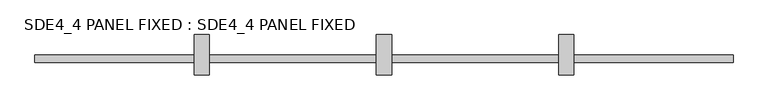
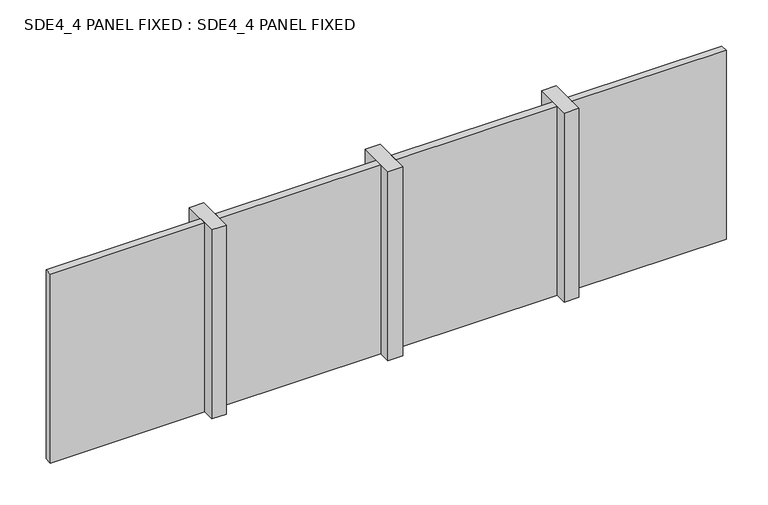
"""IFC4 building model written with IfcOpenShell, lengths in millimetres: plate geometry, SDE4_4 PANEL FIXED : SDE4_4 PANEL FIXED."""

from ifc_helpers import new_model, si_unit, origin, origin_with_axes, place, context, project, spatial, polyline, outline, extrude, source, transform, mapped, element, save


def sde4_4_panel_fixed_sde4_4_panel_fixed_aee83dc5(model_context):
    return source(origin(), model_context, "Body", "SweptSolid", [
        extrude(outline(polyline([(-1150.0, -132.5), (-1250.0, -132.5), (-1250.0, 132.5), (-1150.0, 132.5), (-1150.0, -132.5)])), origin_with_axes(), (0.0, 0.0, 1.0), 1360.0),
        extrude(outline(polyline([(50.0, -132.5), (-50.0, -132.5), (-50.0, 132.5), (50.0, 132.5), (50.0, -132.5)])), origin_with_axes(), (0.0, 0.0, 1.0), 1360.0),
        extrude(outline(polyline([(1250.0, -132.5), (1150.0, -132.5), (1150.0, 132.5), (1250.0, 132.5), (1250.0, -132.5)])), origin_with_axes(), (0.0, 0.0, 1.0), 1360.0),
        extrude(outline(polyline([(2299.0, -50.0), (1250.0, -50.0), (1250.0, 0.0), (2299.0, 0.0), (2299.0, -50.0)])), origin_with_axes(), (0.0, 0.0, 1.0), 1360.0),
        extrude(outline(polyline([(1150.0, -50.0), (50.0, -50.0), (50.0, 0.0), (1150.0, 0.0), (1150.0, -50.0)])), origin_with_axes(), (0.0, 0.0, 1.0), 1360.0),
        extrude(outline(polyline([(-50.0, -50.0), (-1150.0, -50.0), (-1150.0, 0.0), (-50.0, 0.0), (-50.0, -50.0)])), origin_with_axes(), (0.0, 0.0, 1.0), 1360.0),
        extrude(outline(polyline([(-1250.0, -50.0), (-2300.0, -50.0), (-2300.0, 0.0), (-1250.0, 0.0), (-1250.0, -50.0)])), origin_with_axes(), (0.0, 0.0, 1.0), 1360.0),
    ])


if __name__ == "__main__":
    model = new_model("IFC4")
    model_context = context("Model", 3, world=origin())
    ifc_project = project(units=[si_unit("LENGTHUNIT", "METRE", prefix="MILLI")], contexts=[model_context])
    site = spatial("IfcSite", under=ifc_project)
    building = spatial("IfcBuilding", under=site)
    placement = place(None, origin())
    sde4_4_panel_fixed_sde4_4_panel_fixed_shape = sde4_4_panel_fixed_sde4_4_panel_fixed_aee83dc5(model_context)
    element("IfcPlate", 1, ObjectType="SDE4_4 PANEL FIXED : SDE4_4 PANEL FIXED", at=placement, inside=building, context=model_context, shape_type="MappedRepresentation", body=[
        mapped(sde4_4_panel_fixed_sde4_4_panel_fixed_shape, transform((0.0, 0.0, 0.0), x_axis=(1.0, 0.0, 0.0), y_axis=(0.0, 1.0, 0.0), z_axis=(0.0, 0.0, 1.0))),
    ])
    save(model, "model.ifc")

# Revit data of these elements
# Type "SDE4_4 PANEL FIXED : SDE4_4 PANEL FIXED"
#   Type Mark = "CW-GLASS"
#   Analytic Construction = "<None>"
#   Glass = Glass
#   Frame = Aluminium
# Element 1 (IfcPlate, "SDE4_4 PANEL FIXED : SDE4_4 PANEL FIXED")
#   Materials on its faces: "Glass", "Aluminium"
# Materials
#   "Glass": class "Glass", colour RGB 0 128 192, transparency 0.9, Keynote = "L40", Cost = 0
#   "Aluminium": class "Unassigned", colour RGB 247 247 247, transparency 0, Cost = 0
